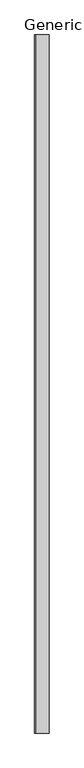
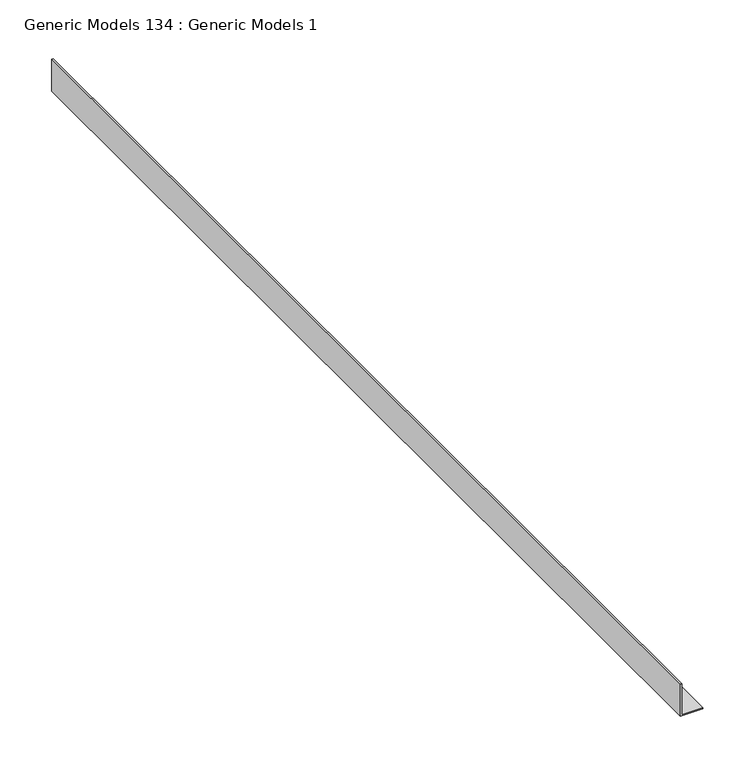
"""IFC4 building model written with IfcOpenShell, lengths in millimetres: proxy geometry, Generic Models 134 : Generic Models 1."""

import ifcopenshell
import ifcopenshell.guid

model = None  # the IFC model being written
_history = None  # IfcOwnerHistory: only IFC2X3 demands one
_inside = {}  # id of a spatial element -> (the spatial element, [elements in it])
_under = {}  # id of a project, library or spatial element -> (it, [spatial elements below it])
_declared = {}  # id of a project -> (the project, [libraries it declares])
_typed = {}  # id of a type object -> (the type object, [elements of that type])
_made_of = {}  # id of a material, layer set ... -> (it, [elements and type objects made of it])


def new_model(schema):
    """Start an empty IFC model of exactly this schema.

    Asked for "IFC4X3", IfcOpenShell would pick the latest addendum, in which some entities
    have other attributes; the version numbers below select the first issue.
    IFC2X3 requires an IfcOwnerHistory on every rooted entity: one is made here for all.
    """
    global model, _history
    if schema == "IFC4X3":
        model = ifcopenshell.file(schema_version=(4, 3, 0, 0))
    else:
        model = ifcopenshell.file(schema=schema)
    _inside.clear()
    _under.clear()
    _declared.clear()
    _typed.clear()
    _made_of.clear()
    _history = None
    if model.schema == "IFC2X3":
        org = make("IfcOrganization", Name="unknown")
        user = make(
            "IfcPersonAndOrganization",
            ThePerson=make("IfcPerson", FamilyName="unknown"),
            TheOrganization=org,
        )
        app = make(
            "IfcApplication",
            ApplicationDeveloper=org,
            Version="unknown",
            ApplicationFullName="unknown",
            ApplicationIdentifier="unknown",
        )
        _history = make(
            "IfcOwnerHistory",
            OwningUser=user,
            OwningApplication=app,
            ChangeAction="ADDED",
            CreationDate=0,
        )
    return model


def make(cls, **values):
    """One entity of the class cls with the attributes given. An attribute that is None is left unset."""
    return model.create_entity(
        cls, **{name: value for name, value in values.items() if value is not None}
    )


def rooted(cls, **values):
    """An entity with a GlobalId (a new one), such as an element, a storey or a relation."""
    return make(cls, GlobalId=ifcopenshell.guid.new(), OwnerHistory=_history, **values)


def si_unit(unit_type, name, prefix=None):
    """IfcSIUnit, for example si_unit("LENGTHUNIT", "METRE", prefix="MILLI")."""
    return make("IfcSIUnit", UnitType=unit_type, Prefix=prefix, Name=name)


def assignment(units):
    """IfcUnitAssignment: the units of a project."""
    return None if units is None else make("IfcUnitAssignment", Units=units)


def point(xyz):
    """IfcCartesianPoint."""
    return None if xyz is None else make("IfcCartesianPoint", Coordinates=xyz)


def direction(xyz):
    """IfcDirection."""
    return None if xyz is None else make("IfcDirection", DirectionRatios=xyz)


def frame(location, z_axis=None, x_axis=None):
    """IfcAxis2Placement3D, a coordinate frame: its origin and axes. An axis left out is left unset."""
    return make(
        "IfcAxis2Placement3D",
        Location=point(location),
        Axis=direction(z_axis),
        RefDirection=direction(x_axis),
    )


def origin():
    """The frame at (0, 0, 0) with its axes left unset."""
    return frame((0.0, 0.0, 0.0))


def place(relative_to, where):
    """IfcLocalPlacement: puts the frame where relative to a parent placement (None: the world)."""
    return make(
        "IfcLocalPlacement", PlacementRelTo=relative_to, RelativePlacement=where
    )


def context(
    kind, dimensions, precision=None, world=None, true_north=None, identifier=None
):
    """IfcGeometricRepresentationContext, for example the 3D "Model" context."""
    return make(
        "IfcGeometricRepresentationContext",
        ContextIdentifier=identifier,
        ContextType=kind,
        CoordinateSpaceDimension=dimensions,
        Precision=precision,
        WorldCoordinateSystem=world,
        TrueNorth=true_north,
    )


def project(units=None, contexts=None):
    """IfcProject with its units and contexts."""
    return rooted(
        "IfcProject",
        Name="project",
        RepresentationContexts=contexts,
        UnitsInContext=assignment(units),
    )


def spatial(cls, under=None, at=None, **own):
    """A site, building, storey or space (cls), placed at a placement, below another one or the project."""
    s = rooted(cls, ObjectPlacement=at, **own)
    if under is not None:
        _under.setdefault(under.id(), (under, []))[1].append(s)
    return s


def polyline(points):
    """IfcPolyline through the points."""
    return make("IfcPolyline", Points=[point(p) for p in points])


def outline(outer, holes=None, kind="AREA"):
    """IfcArbitraryClosedProfileDef: a profile drawn as a closed curve; with holes, ...WithVoids."""
    if holes is None:
        return make("IfcArbitraryClosedProfileDef", ProfileType=kind, OuterCurve=outer)
    return make(
        "IfcArbitraryProfileDefWithVoids",
        ProfileType=kind,
        OuterCurve=outer,
        InnerCurves=holes,
    )


def extrude(swept, where, along, depth):
    """IfcExtrudedAreaSolid: the profile swept, set in the frame where, extruded along a direction by depth."""
    return make(
        "IfcExtrudedAreaSolid",
        SweptArea=swept,
        Position=where,
        ExtrudedDirection=direction(along),
        Depth=depth,
    )


def shape(context_of_items, identifier, shape_type, items):
    """IfcShapeRepresentation: the items that make up one representation, for example the "Body"."""
    return make(
        "IfcShapeRepresentation",
        ContextOfItems=context_of_items,
        RepresentationIdentifier=identifier,
        RepresentationType=shape_type,
        Items=items,
    )


def source(mapping_origin, context_of_items, identifier, shape_type, items):
    """IfcRepresentationMap: a shape defined once, which mapped items show again and again."""
    return make(
        "IfcRepresentationMap",
        MappingOrigin=mapping_origin,
        MappedRepresentation=shape(context_of_items, identifier, shape_type, items),
    )


def transform(
    local_origin,
    x_axis=None,
    y_axis=None,
    z_axis=None,
    scale=None,
    scale2=None,
    scale3=None,
    uniform=True,
):
    """IfcCartesianTransformationOperator3D, or its non-uniform kind. x_axis, y_axis, z_axis: its Axis1, 2, 3."""
    if uniform:
        return make(
            "IfcCartesianTransformationOperator3D",
            Axis1=direction(x_axis),
            Axis2=direction(y_axis),
            LocalOrigin=point(local_origin),
            Scale=scale,
            Axis3=direction(z_axis),
        )
    return make(
        "IfcCartesianTransformationOperator3DnonUniform",
        Axis1=direction(x_axis),
        Axis2=direction(y_axis),
        LocalOrigin=point(local_origin),
        Scale=scale,
        Axis3=direction(z_axis),
        Scale2=scale2,
        Scale3=scale3,
    )


def mapped(mapping_source, mapping_target):
    """IfcMappedItem: shows the shape of a source again, moved by a transform."""
    return make(
        "IfcMappedItem", MappingSource=mapping_source, MappingTarget=mapping_target
    )


def made_of(thing, what):
    """Note that an element or type object is made of a material, layer set ...; save() writes the relation."""
    if what is not None:
        _made_of.setdefault(what.id(), (what, []))[1].append(thing)
    return thing


def element(
    cls,
    number,
    at=None,
    inside=None,
    cuts=None,
    type_object=None,
    material=None,
    context=None,
    identifier="Body",
    shape_type=None,
    held_by="IfcProductDefinitionShape",
    body=None,
    shapes=None,
    **own,
):
    """One element of the class cls, such as IfcWall. Its Tag is "e" and its number.

    at: its placement. inside: the storey or other place that contains it. cuts: it is an
    opening in that element (IfcRelVoidsElement). A single representation is given by context,
    identifier, shape_type and body (its items); several are given by shapes. held_by: the class
    of the entity that holds the representations. save() writes the other relations.
    """
    e = rooted(cls, Tag="e%d" % number, ObjectPlacement=at, **own)
    if body is not None:
        shapes = [shape(context, identifier, shape_type, body)]
    if shapes is not None:
        e.Representation = make(held_by, Representations=shapes)
    if inside is not None:
        _inside.setdefault(inside.id(), (inside, []))[1].append(e)
    if cuts is not None:
        rooted(
            "IfcRelVoidsElement", RelatingBuildingElement=cuts, RelatedOpeningElement=e
        )
    if type_object is not None:
        _typed.setdefault(type_object.id(), (type_object, []))[1].append(e)
    return made_of(e, material)


def aggregate(whole, parts):
    """IfcRelAggregates: a whole, such as a stair, and the parts it consists of."""
    return rooted("IfcRelAggregates", RelatingObject=whole, RelatedObjects=parts)


def save(model, path):
    """Write the relations noted so far, then the file.

    IfcRelAggregates (storeys below a building ...), IfcRelContainedInSpatialStructure (elements
    in a storey), IfcRelDefinesByType, IfcRelAssociatesMaterial and IfcRelDeclares: one each for
    every whole, place, type object, material and project.
    """
    for whole, parts in _under.values():
        aggregate(whole, parts)
    for where, things in _inside.values():
        rooted(
            "IfcRelContainedInSpatialStructure",
            RelatedElements=things,
            RelatingStructure=where,
        )
    for kind, things in _typed.values():
        rooted("IfcRelDefinesByType", RelatedObjects=things, RelatingType=kind)
    for what, things in _made_of.values():
        rooted("IfcRelAssociatesMaterial", RelatedObjects=things, RelatingMaterial=what)
    for by, libraries in _declared.values():
        rooted("IfcRelDeclares", RelatingContext=by, RelatedDefinitions=libraries)
    model.write(path)


def generic_models_134_generic_models_1_20abfd65(model_context):
    return source(origin(), model_context, "Body", "SweptSolid", [
        extrude(outline(polyline([(126.6971102, 49818.1931639), (88.5971102, 49818.1931639), (88.5971102, 49843.5931639), (90.1846102, 49843.5931639), (90.1846102, 49819.7806639), (126.6971102, 49819.7806639), (126.6971102, 49818.1931639)])), frame((0.0, 0.0, 0.0), z_axis=(0.0, 1.0, 0.0), x_axis=(0.0, 0.0, 1.0)), (0.0, 0.0, 1.0), 1219.2),
    ])


if __name__ == "__main__":
    model = new_model("IFC4")
    model_context = context("Model", 3, world=origin())
    ifc_project = project(units=[si_unit("LENGTHUNIT", "METRE", prefix="MILLI")], contexts=[model_context])
    site = spatial("IfcSite", under=ifc_project)
    building = spatial("IfcBuilding", under=site)
    placement = place(None, origin())
    generic_models_134_generic_models_1_shape = generic_models_134_generic_models_1_20abfd65(model_context)
    element("IfcBuildingElementProxy", 1, Name="Generic Models 134 : Generic Models 1", ObjectType="Generic Models 134 : Generic Models 1", at=placement, inside=building, context=model_context, shape_type="MappedRepresentation", body=[
        mapped(generic_models_134_generic_models_1_shape, transform((0.0, 0.0, 0.0), x_axis=(1.0, 0.0, 0.0), y_axis=(0.0, 1.0, 0.0), z_axis=(0.0, 0.0, 1.0))),
    ])
    save(model, "model.ifc")

# Revit data of these elements
# Element 1 (IfcBuildingElementProxy, "Generic Models 134 : Generic Models 1")
#   Materials on its faces: "CEILING TRACK TO MATCH EXISTING"
# Materials
#   "CEILING TRACK TO MATCH EXISTING": class "Unassigned", colour RGB 210 209 208, transparency 0, Keynote = "M05121300.02", Cost = 0
